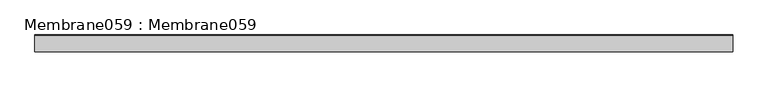
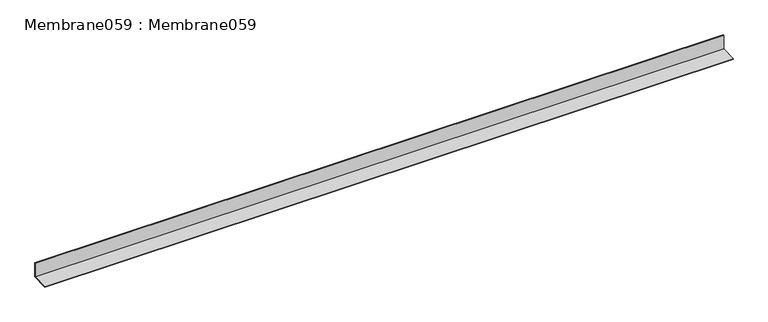
"""IFC4 building model written with IfcOpenShell, lengths in millimetres: proxy geometry, Membrane059 : Membrane059."""

from ifc_helpers import new_model, si_unit, frame, origin, place, context, project, spatial, polyline, outline, extrude, source, transform, mapped, element, save


def membrane059_membrane059_eccd656e(model_context):
    return source(origin(), model_context, "Body", "SweptSolid", [
        extrude(outline(polyline([(-4411.6511719, 40279.5078125), (-4410.4511719, 40279.5078125), (-4410.4511719, 40236.265625), (-4459.1279297, 40234.9804688), (-4459.1596009, 40236.1800507), (-4411.6511719, 40237.4343609), (-4411.6511719, 40279.5078125)])), frame((12383.0178845, 0.0, 0.0), z_axis=(1.0, 0.0, 0.0), x_axis=(0.0, 1.0, 0.0)), (0.0, 0.0, 1.0), 2000.0),
    ])


if __name__ == "__main__":
    model = new_model("IFC4")
    model_context = context("Model", 3, world=origin())
    ifc_project = project(units=[si_unit("LENGTHUNIT", "METRE", prefix="MILLI")], contexts=[model_context])
    site = spatial("IfcSite", under=ifc_project)
    building = spatial("IfcBuilding", under=site)
    placement = place(None, origin())
    membrane059_membrane059_shape = membrane059_membrane059_eccd656e(model_context)
    element("IfcBuildingElementProxy", 1, Name="Membrane059 : Membrane059", ObjectType="Membrane059 : Membrane059", at=placement, inside=building, context=model_context, shape_type="MappedRepresentation", body=[
        mapped(membrane059_membrane059_shape, transform((0.0, 0.0, 0.0), x_axis=(1.0, 0.0, 0.0), y_axis=(0.0, 1.0, 0.0), z_axis=(0.0, 0.0, 1.0))),
    ])
    save(model, "model.ifc")

# Revit data of these elements
# Type "Membrane059 : Membrane059"
#   NameOverride = "Membrane059"
# Element 1 (IfcBuildingElementProxy, "Membrane059 : Membrane059")
#   Materials on its faces: "2 LAYERS NO. 30 ASTM D226 ASPHALT SATURATED ORGANIC FELT"
# Materials
#   "2 LAYERS NO. 30 ASTM D226 ASPHALT SATURATED ORGANIC FELT": class "Unassigned", colour RGB 46 171 0, transparency 0
